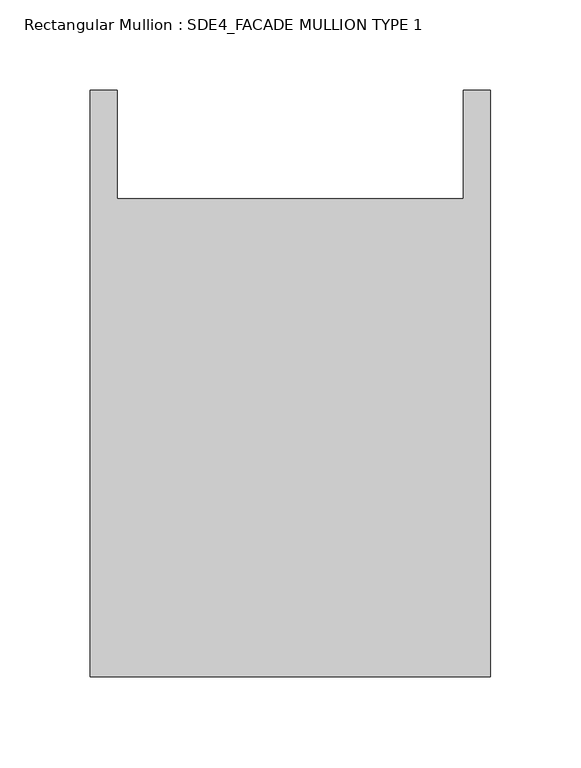
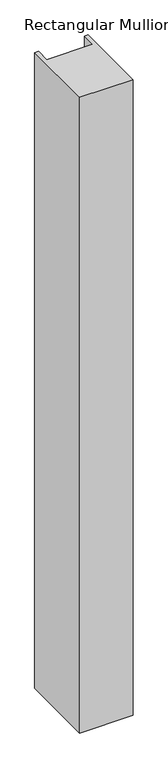
"""IFC4 building model written with IfcOpenShell, lengths in millimetres: member geometry, Rectangular Mullion : SDE4_FACADE MULLION TYPE 1."""

from ifc_helpers import new_model, si_unit, frame, origin, place, context, project, spatial, polyline, outline, extrude, source, transform, mapped, element, save


def rectangular_mullion_sde4_facade_mullion_type_1_80b4d5c7(model_context):
    return source(origin(), model_context, "Body", "SweptSolid", [
        extrude(outline(polyline([(111.0, -132.5), (-111.0, -132.5), (-111.0, 192.5), (-96.0, 192.5), (-96.0, 132.5), (96.0, 132.5), (96.0, 192.5), (111.0, 192.5), (111.0, -132.5)])), frame((0.0, 0.0, -2800.0), z_axis=(0.0, 0.0, 1.0), x_axis=(1.0, 0.0, 0.0)), (0.0, 0.0, 1.0), 2800.0),
    ])


if __name__ == "__main__":
    model = new_model("IFC4")
    model_context = context("Model", 3, world=origin())
    ifc_project = project(units=[si_unit("LENGTHUNIT", "METRE", prefix="MILLI")], contexts=[model_context])
    site = spatial("IfcSite", under=ifc_project)
    building = spatial("IfcBuilding", under=site)
    placement = place(None, origin())
    rectangular_mullion_sde4_facade_mullion_type_1_shape = rectangular_mullion_sde4_facade_mullion_type_1_80b4d5c7(model_context)
    element("IfcMember", 1, ObjectType="Rectangular Mullion : SDE4_FACADE MULLION TYPE 1", at=placement, inside=building, context=model_context, shape_type="MappedRepresentation", body=[
        mapped(rectangular_mullion_sde4_facade_mullion_type_1_shape, transform((0.0, 0.0, 0.0), x_axis=(1.0, 0.0, 0.0), y_axis=(0.0, 1.0, 0.0), z_axis=(0.0, 0.0, 1.0))),
    ])
    save(model, "model.ifc")

# Revit data of these elements
# Type "Rectangular Mullion : SDE4_FACADE MULLION TYPE 1"
#   built-in parameter 1007322 = 0.869423 (stored number, unit not read)
#   built-in parameter 1007321 = 0.364173 (stored number, unit not read)
#   built-in parameter 1007320 = 0.364173 (stored number, unit not read)
